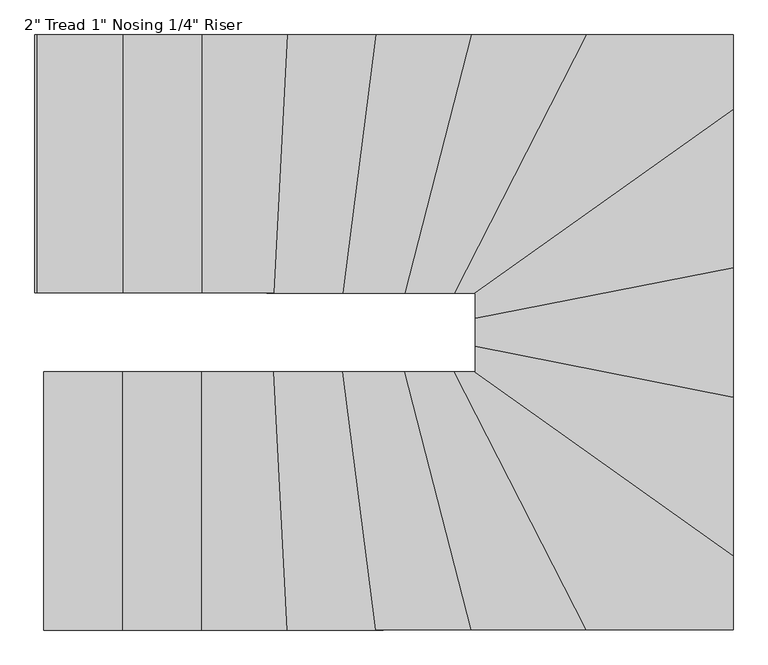
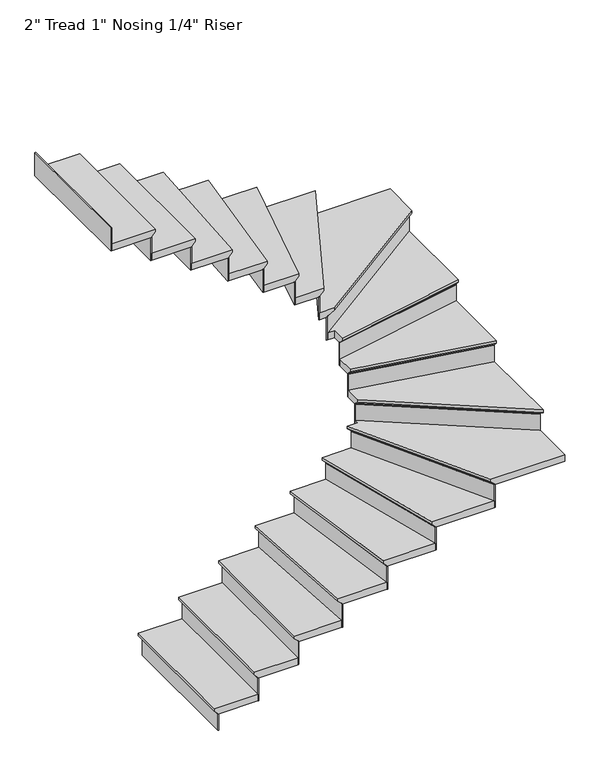
"""IFC4 building model written with IfcOpenShell, lengths in millimetres: stair flight geometry."""

import ifcopenshell
import ifcopenshell.guid

model = None  # the IFC model being written
_history = None  # IfcOwnerHistory: only IFC2X3 demands one
_inside = {}  # id of a spatial element -> (the spatial element, [elements in it])
_under = {}  # id of a project, library or spatial element -> (it, [spatial elements below it])
_declared = {}  # id of a project -> (the project, [libraries it declares])
_typed = {}  # id of a type object -> (the type object, [elements of that type])
_made_of = {}  # id of a material, layer set ... -> (it, [elements and type objects made of it])


def new_model(schema):
    """Start an empty IFC model of exactly this schema.

    Asked for "IFC4X3", IfcOpenShell would pick the latest addendum, in which some entities
    have other attributes; the version numbers below select the first issue.
    IFC2X3 requires an IfcOwnerHistory on every rooted entity: one is made here for all.
    """
    global model, _history
    if schema == "IFC4X3":
        model = ifcopenshell.file(schema_version=(4, 3, 0, 0))
    else:
        model = ifcopenshell.file(schema=schema)
    _inside.clear()
    _under.clear()
    _declared.clear()
    _typed.clear()
    _made_of.clear()
    _history = None
    if model.schema == "IFC2X3":
        org = make("IfcOrganization", Name="unknown")
        user = make(
            "IfcPersonAndOrganization",
            ThePerson=make("IfcPerson", FamilyName="unknown"),
            TheOrganization=org,
        )
        app = make(
            "IfcApplication",
            ApplicationDeveloper=org,
            Version="unknown",
            ApplicationFullName="unknown",
            ApplicationIdentifier="unknown",
        )
        _history = make(
            "IfcOwnerHistory",
            OwningUser=user,
            OwningApplication=app,
            ChangeAction="ADDED",
            CreationDate=0,
        )
    return model


def make(cls, **values):
    """One entity of the class cls with the attributes given. An attribute that is None is left unset."""
    return model.create_entity(
        cls, **{name: value for name, value in values.items() if value is not None}
    )


def rooted(cls, **values):
    """An entity with a GlobalId (a new one), such as an element, a storey or a relation."""
    return make(cls, GlobalId=ifcopenshell.guid.new(), OwnerHistory=_history, **values)


def si_unit(unit_type, name, prefix=None):
    """IfcSIUnit, for example si_unit("LENGTHUNIT", "METRE", prefix="MILLI")."""
    return make("IfcSIUnit", UnitType=unit_type, Prefix=prefix, Name=name)


def assignment(units):
    """IfcUnitAssignment: the units of a project."""
    return None if units is None else make("IfcUnitAssignment", Units=units)


def point(xyz):
    """IfcCartesianPoint."""
    return None if xyz is None else make("IfcCartesianPoint", Coordinates=xyz)


def direction(xyz):
    """IfcDirection."""
    return None if xyz is None else make("IfcDirection", DirectionRatios=xyz)


def frame(location, z_axis=None, x_axis=None):
    """IfcAxis2Placement3D, a coordinate frame: its origin and axes. An axis left out is left unset."""
    return make(
        "IfcAxis2Placement3D",
        Location=point(location),
        Axis=direction(z_axis),
        RefDirection=direction(x_axis),
    )


def origin():
    """The frame at (0, 0, 0) with its axes left unset."""
    return frame((0.0, 0.0, 0.0))


def place(relative_to, where):
    """IfcLocalPlacement: puts the frame where relative to a parent placement (None: the world)."""
    return make(
        "IfcLocalPlacement", PlacementRelTo=relative_to, RelativePlacement=where
    )


def context(
    kind, dimensions, precision=None, world=None, true_north=None, identifier=None
):
    """IfcGeometricRepresentationContext, for example the 3D "Model" context."""
    return make(
        "IfcGeometricRepresentationContext",
        ContextIdentifier=identifier,
        ContextType=kind,
        CoordinateSpaceDimension=dimensions,
        Precision=precision,
        WorldCoordinateSystem=world,
        TrueNorth=true_north,
    )


def project(units=None, contexts=None):
    """IfcProject with its units and contexts."""
    return rooted(
        "IfcProject",
        Name="project",
        RepresentationContexts=contexts,
        UnitsInContext=assignment(units),
    )


def spatial(cls, under=None, at=None, **own):
    """A site, building, storey or space (cls), placed at a placement, below another one or the project."""
    s = rooted(cls, ObjectPlacement=at, **own)
    if under is not None:
        _under.setdefault(under.id(), (under, []))[1].append(s)
    return s


def faces_of(points, faces, orient=None, outer=None):
    """IfcFace entities. A face is a list of loops; a loop is a list of indices into points, from 0.

    orient and outer hold one flag for each loop. By default every Orientation is true, the
    first loop of a face is its IfcFaceOuterBound and the others are IfcFaceBound.
    """
    made = []
    for i, loops in enumerate(faces):
        bounds = []
        for j, loop in enumerate(loops):
            is_outer = j == 0 if outer is None else outer[i][j]
            bounds.append(
                make(
                    "IfcFaceOuterBound" if is_outer else "IfcFaceBound",
                    Bound=make("IfcPolyLoop", Polygon=[points[k] for k in loop]),
                    Orientation=True if orient is None else orient[i][j],
                )
            )
        made.append(make("IfcFace", Bounds=bounds))
    return made


def faceted_brep(points, faces, orient=None, outer=None, voids=None):
    """IfcFacetedBrep: a solid bounded by flat faces; with voids (closed shells), ...WithVoids."""
    shared = [point(p) for p in points]
    hull = make("IfcClosedShell", CfsFaces=faces_of(shared, faces, orient, outer))
    if voids is None:
        return make("IfcFacetedBrep", Outer=hull)
    return make(
        "IfcFacetedBrepWithVoids",
        Outer=hull,
        Voids=[
            make(cls, CfsFaces=faces_of(shared, fs, o, b)) for cls, fs, o, b in voids
        ],
    )


def shape(context_of_items, identifier, shape_type, items):
    """IfcShapeRepresentation: the items that make up one representation, for example the "Body"."""
    return make(
        "IfcShapeRepresentation",
        ContextOfItems=context_of_items,
        RepresentationIdentifier=identifier,
        RepresentationType=shape_type,
        Items=items,
    )


def source(mapping_origin, context_of_items, identifier, shape_type, items):
    """IfcRepresentationMap: a shape defined once, which mapped items show again and again."""
    return make(
        "IfcRepresentationMap",
        MappingOrigin=mapping_origin,
        MappedRepresentation=shape(context_of_items, identifier, shape_type, items),
    )


def transform(
    local_origin,
    x_axis=None,
    y_axis=None,
    z_axis=None,
    scale=None,
    scale2=None,
    scale3=None,
    uniform=True,
):
    """IfcCartesianTransformationOperator3D, or its non-uniform kind. x_axis, y_axis, z_axis: its Axis1, 2, 3."""
    if uniform:
        return make(
            "IfcCartesianTransformationOperator3D",
            Axis1=direction(x_axis),
            Axis2=direction(y_axis),
            LocalOrigin=point(local_origin),
            Scale=scale,
            Axis3=direction(z_axis),
        )
    return make(
        "IfcCartesianTransformationOperator3DnonUniform",
        Axis1=direction(x_axis),
        Axis2=direction(y_axis),
        LocalOrigin=point(local_origin),
        Scale=scale,
        Axis3=direction(z_axis),
        Scale2=scale2,
        Scale3=scale3,
    )


def mapped(mapping_source, mapping_target):
    """IfcMappedItem: shows the shape of a source again, moved by a transform."""
    return make(
        "IfcMappedItem", MappingSource=mapping_source, MappingTarget=mapping_target
    )


def made_of(thing, what):
    """Note that an element or type object is made of a material, layer set ...; save() writes the relation."""
    if what is not None:
        _made_of.setdefault(what.id(), (what, []))[1].append(thing)
    return thing


def element(
    cls,
    number,
    at=None,
    inside=None,
    cuts=None,
    type_object=None,
    material=None,
    context=None,
    identifier="Body",
    shape_type=None,
    held_by="IfcProductDefinitionShape",
    body=None,
    shapes=None,
    **own,
):
    """One element of the class cls, such as IfcWall. Its Tag is "e" and its number.

    at: its placement. inside: the storey or other place that contains it. cuts: it is an
    opening in that element (IfcRelVoidsElement). A single representation is given by context,
    identifier, shape_type and body (its items); several are given by shapes. held_by: the class
    of the entity that holds the representations. save() writes the other relations.
    """
    e = rooted(cls, Tag="e%d" % number, ObjectPlacement=at, **own)
    if body is not None:
        shapes = [shape(context, identifier, shape_type, body)]
    if shapes is not None:
        e.Representation = make(held_by, Representations=shapes)
    if inside is not None:
        _inside.setdefault(inside.id(), (inside, []))[1].append(e)
    if cuts is not None:
        rooted(
            "IfcRelVoidsElement", RelatingBuildingElement=cuts, RelatedOpeningElement=e
        )
    if type_object is not None:
        _typed.setdefault(type_object.id(), (type_object, []))[1].append(e)
    return made_of(e, material)


def aggregate(whole, parts):
    """IfcRelAggregates: a whole, such as a stair, and the parts it consists of."""
    return rooted("IfcRelAggregates", RelatingObject=whole, RelatedObjects=parts)


def save(model, path):
    """Write the relations noted so far, then the file.

    IfcRelAggregates (storeys below a building ...), IfcRelContainedInSpatialStructure (elements
    in a storey), IfcRelDefinesByType, IfcRelAssociatesMaterial and IfcRelDeclares: one each for
    every whole, place, type object, material and project.
    """
    for whole, parts in _under.values():
        aggregate(whole, parts)
    for where, things in _inside.values():
        rooted(
            "IfcRelContainedInSpatialStructure",
            RelatedElements=things,
            RelatingStructure=where,
        )
    for kind, things in _typed.values():
        rooted("IfcRelDefinesByType", RelatedObjects=things, RelatingType=kind)
    for what, things in _made_of.values():
        rooted("IfcRelAssociatesMaterial", RelatedObjects=things, RelatingMaterial=what)
    for by, libraries in _declared.values():
        rooted("IfcRelDeclares", RelatingContext=by, RelatedDefinitions=libraries)
    model.write(path)


def stair_flight_c1eb027c(model_context):
    return source(origin(), model_context, "Body", "Brep", [
        faceted_brep([(-16321.7832832, 2938.4294183, 150.2833333), (-16321.7832832, 2938.4294183, 169.3333333), (-16321.7832832, 3852.8294183, 169.3333333), (-16321.7832832, 3852.8294183, 150.2833333), (-16296.3832832, 2938.4294183, 124.8833333), (-16296.3832832, 3852.8294183, 124.8833333), (-16016.9832832, 2938.4294183, 169.3333333), (-16016.9832832, 3852.8294183, 169.3333333), (-16296.3832832, 3852.8294183, 118.5333333), (-16016.9832832, 3852.8294183, 118.5333333), (-16016.9832832, 2938.4294183, 118.5333333), (-16296.3832832, 2938.4294183, 118.5333333)], [[[0, 1, 2, 3]], [[4, 0, 3, 5]], [[2, 1, 6, 7]], [[8, 9, 10, 11]], [[2, 7, 9, 8, 5, 3]], [[8, 11, 4, 5]], [[6, 1, 0, 4, 11, 10]], [[7, 6, 10, 9]]]),
        faceted_brep([(-16296.3832832, 2938.4294183, 118.5333333), (-16296.3832832, 2938.4294183, 0.0), (-16290.0332832, 2938.4294183, 0.0), (-16290.0332832, 2938.4294183, 118.5333333), (-16296.3832832, 3852.8294183, 118.5333333), (-16290.0332832, 3852.8294183, 118.5333333), (-16290.0332832, 3852.8294183, 0.0), (-16296.3832832, 3852.8294183, 0.0)], [[[0, 1, 2, 3]], [[4, 5, 6, 7]], [[1, 0, 4, 7]], [[2, 1, 7, 6]], [[3, 2, 6, 5]], [[0, 3, 5, 4]]]),
        faceted_brep([(-16016.9832832, 2938.4294183, 287.8666667), (-16016.9832832, 2938.4294183, 118.5333333), (-16010.6332832, 2938.4294183, 118.5333333), (-16010.6332832, 2938.4294183, 287.8666667), (-16016.9832832, 3852.8294183, 287.8666667), (-16010.6332832, 3852.8294183, 287.8666667), (-16010.6332832, 3852.8294183, 118.5333333), (-16016.9832832, 3852.8294183, 118.5333333)], [[[0, 1, 2, 3]], [[4, 5, 6, 7]], [[1, 0, 4, 7]], [[2, 1, 7, 6]], [[3, 2, 6, 5]], [[0, 3, 5, 4]]]),
        faceted_brep([(-16042.3832832, 3852.8294183, 338.6666667), (-16042.3832832, 2938.4294183, 338.6666667), (-15737.5832832, 2938.4294183, 338.6666667), (-15737.5832832, 3852.8294183, 338.6666667), (-16016.9832832, 3852.8294183, 287.8666667), (-15737.5832832, 3852.8294183, 287.8666667), (-15737.5832832, 2938.4294183, 287.8666667), (-16016.9832832, 2938.4294183, 287.8666667), (-16016.9832832, 3852.8294183, 294.2166667), (-16042.3832832, 3852.8294183, 319.6166667), (-16016.9832832, 2938.4294183, 294.2166667), (-16042.3832832, 2938.4294183, 319.6166667)], [[[0, 1, 2, 3]], [[4, 5, 6, 7]], [[0, 3, 5, 4, 8, 9]], [[4, 7, 10, 8]], [[2, 1, 11, 10, 7, 6]], [[3, 2, 6, 5]], [[11, 1, 0, 9]], [[10, 11, 9, 8]]]),
        faceted_brep([(-15737.5832832, 2938.4294183, 457.2), (-15737.5832832, 2938.4294183, 287.8666667), (-15731.2332832, 2938.4294183, 287.8666667), (-15731.2332832, 2938.4294183, 457.2), (-15737.5832832, 3852.8294183, 457.2), (-15731.2332832, 3852.8294183, 457.2), (-15731.2332832, 3852.8294183, 287.8666667), (-15737.5832832, 3852.8294183, 287.8666667)], [[[0, 1, 2, 3]], [[4, 5, 6, 7]], [[1, 0, 4, 7]], [[2, 1, 7, 6]], [[3, 2, 6, 5]], [[0, 3, 5, 4]]]),
        faceted_brep([(-15762.9832832, 3852.8294183, 508.0), (-15762.9832832, 2938.4294183, 508.0), (-15434.3818513, 2938.4294183, 508.0), (-15481.9161218, 3852.8294183, 508.0), (-15737.5832832, 3852.8294183, 457.2), (-15481.9161218, 3852.8294183, 457.2), (-15434.3818513, 2938.4294183, 457.2), (-15737.5832832, 2938.4294183, 457.2), (-15737.5832832, 3852.8294183, 463.55), (-15762.9832832, 3852.8294183, 488.95), (-15737.5832832, 2938.4294183, 463.55), (-15762.9832832, 2938.4294183, 488.95)], [[[0, 1, 2, 3]], [[4, 5, 6, 7]], [[0, 3, 5, 4, 8, 9]], [[4, 7, 10, 8]], [[2, 1, 11, 10, 7, 6]], [[3, 2, 6, 5]], [[11, 1, 0, 9]], [[10, 11, 9, 8]]]),
        faceted_brep([(-15434.3818513, 2938.4294183, 626.5333333), (-15434.3818513, 2938.4294183, 457.2), (-15428.0232772, 2938.4294183, 457.2), (-15428.0232772, 2938.4294183, 626.5333333), (-15481.9161218, 3852.8294183, 626.5333333), (-15475.5575476, 3852.8294183, 626.5333333), (-15475.5575476, 3852.8294183, 457.2), (-15481.9161218, 3852.8294183, 457.2)], [[[0, 1, 2, 3]], [[4, 5, 6, 7]], [[1, 0, 4, 7]], [[2, 1, 7, 6]], [[3, 2, 6, 5]], [[0, 3, 5, 4]]]),
        faceted_brep([(-15507.3504184, 3852.8294183, 677.3333333), (-15459.816148, 2938.4294183, 677.3333333), (-15119.3933703, 2938.4294183, 677.3333333), (-15237.7494219, 3852.8294183, 677.3333333), (-15481.9161218, 3852.8294183, 626.5333333), (-15237.7494219, 3852.8294183, 626.5333333), (-15119.3933703, 2938.4294183, 626.5333333), (-15434.3818513, 2938.4294183, 626.5333333), (-15481.9161218, 3852.8294183, 632.8833333), (-15507.3504184, 3852.8294183, 658.2833333), (-15434.3818513, 2938.4294183, 632.8833333), (-15459.816148, 2938.4294183, 658.2833333)], [[[0, 1, 2, 3]], [[4, 5, 6, 7]], [[0, 3, 5, 4, 8, 9]], [[4, 7, 10, 8]], [[2, 1, 11, 10, 7, 6]], [[3, 2, 6, 5]], [[11, 1, 0, 9]], [[10, 11, 9, 8]]]),
        faceted_brep([(-15119.3933703, 2938.4294183, 795.8666667), (-15119.3933703, 2938.4294183, 626.5333333), (-15112.9903985, 2938.4294183, 626.5333333), (-15112.9903985, 2938.4294183, 795.8666667), (-15237.7494219, 3852.8294183, 795.8666667), (-15231.3464501, 3852.8294183, 795.8666667), (-15231.3464501, 3852.8294183, 626.5333333), (-15237.7494219, 3852.8294183, 626.5333333)], [[[0, 1, 2, 3]], [[4, 5, 6, 7]], [[1, 0, 4, 7]], [[2, 1, 7, 6]], [[3, 2, 6, 5]], [[0, 3, 5, 4]]]),
        faceted_brep([(-15263.361309, 3852.8294183, 846.6666667), (-15145.0052574, 2938.4294183, 846.6666667), (-14780.991752, 2938.4294183, 846.6666667), (-15016.1221995, 3852.8294183, 846.6666667), (-15237.7494219, 3852.8294183, 795.8666667), (-15016.1221995, 3852.8294183, 795.8666667), (-14780.991752, 2938.4294183, 795.8666667), (-15119.3933703, 2938.4294183, 795.8666667), (-15237.7494219, 3852.8294183, 802.2166667), (-15263.361309, 3852.8294183, 827.6166667), (-15119.3933703, 2938.4294183, 802.2166667), (-15145.0052574, 2938.4294183, 827.6166667)], [[[0, 1, 2, 3]], [[4, 5, 6, 7]], [[0, 3, 5, 4, 8, 9]], [[4, 7, 10, 8]], [[2, 1, 11, 10, 7, 6]], [[3, 2, 6, 5]], [[11, 1, 0, 9]], [[10, 11, 9, 8]]]),
        faceted_brep([(-14780.991752, 2938.4294183, 965.2), (-14780.991752, 2938.4294183, 795.8666667), (-14774.4351752, 2938.4294183, 795.8666667), (-14774.4351752, 2938.4294183, 965.2), (-15016.1221995, 3852.8294183, 965.2), (-15009.5656226, 3852.8294183, 965.2), (-15009.5656226, 3852.8294183, 795.8666667), (-15016.1221995, 3852.8294183, 795.8666667)], [[[0, 1, 2, 3]], [[4, 5, 6, 7]], [[1, 0, 4, 7]], [[2, 1, 7, 6]], [[3, 2, 6, 5]], [[0, 3, 5, 4]]]),
        faceted_brep([(-15042.3485069, 3852.8294183, 1016.0), (-14807.2180595, 2938.4294183, 1016.0), (-14370.950942, 2938.4294183, 1016.0), (-14839.7755634, 3852.8294183, 1016.0), (-15016.1221995, 3852.8294183, 965.2), (-14839.7755634, 3852.8294183, 965.2), (-14370.950942, 2938.4294183, 965.2), (-14780.991752, 2938.4294183, 965.2), (-15016.1221995, 3852.8294183, 971.55), (-15042.3485069, 3852.8294183, 996.95), (-14780.991752, 2938.4294183, 971.55), (-14807.2180595, 2938.4294183, 996.95)], [[[0, 1, 2, 3]], [[4, 5, 6, 7]], [[0, 3, 5, 4, 8, 9]], [[4, 7, 10, 8]], [[2, 1, 11, 10, 7, 6]], [[3, 2, 6, 5]], [[11, 1, 0, 9]], [[10, 11, 9, 8]]]),
        faceted_brep([(-14370.950942, 2938.4294183, 1134.5333333), (-14370.950942, 2938.4294183, 965.2), (-14363.8149589, 2938.4294183, 965.2), (-14363.8149589, 2938.4294183, 1134.5333333), (-14839.7755634, 3852.8294183, 1134.5333333), (-14832.6395802, 3852.8294183, 1134.5333333), (-14832.6395802, 3852.8294183, 965.2), (-14839.7755634, 3852.8294183, 965.2)], [[[0, 1, 2, 3]], [[4, 5, 6, 7]], [[1, 0, 4, 7]], [[2, 1, 7, 6]], [[3, 2, 6, 5]], [[0, 3, 5, 4]]]),
        faceted_brep([(-14794.0515914, 3882.3845011, 1185.3333333), (-14794.0515914, 3852.8294183, 1185.3333333), (-14868.3194959, 3852.8294183, 1185.3333333), (-14399.4948746, 2938.4294183, 1185.3333333), (-13879.6515914, 2938.4294183, 1185.3333333), (-13879.6515914, 3232.110552, 1185.3333333), (-14794.0515914, 3852.8294183, 1134.5333333), (-14794.0515914, 3882.3845011, 1134.5333333), (-13879.6515914, 3232.110552, 1134.5333333), (-13879.6515914, 2938.4294183, 1134.5333333), (-14370.950942, 2938.4294183, 1134.5333333), (-14839.7755634, 3852.8294183, 1134.5333333), (-14839.7755634, 3852.8294183, 1140.8833333), (-14868.3194959, 3852.8294183, 1166.2833333), (-14370.950942, 2938.4294183, 1140.8833333), (-14399.4948746, 2938.4294183, 1166.2833333)], [[[0, 1, 2, 3, 4, 5]], [[6, 7, 8, 9, 10, 11]], [[1, 0, 7, 6]], [[2, 1, 6, 11, 12, 13]], [[11, 10, 14, 12]], [[4, 3, 15, 14, 10, 9]], [[5, 4, 9, 8]], [[0, 5, 8, 7]], [[15, 3, 2, 13]], [[14, 15, 13, 12]]]),
        faceted_brep([(-13879.6515914, 3232.110552, 1303.8666667), (-13879.6515914, 3232.110552, 1134.5333333), (-13879.6515914, 3239.9025268, 1134.5333333), (-13879.6515914, 3239.9025268, 1303.8666667), (-14794.0515914, 3882.3845011, 1303.8666667), (-14794.0515914, 3890.1764759, 1303.8666667), (-14794.0515914, 3890.1764759, 1134.5333333), (-14794.0515914, 3882.3845011, 1134.5333333)], [[[0, 1, 2, 3]], [[4, 5, 6, 7]], [[1, 0, 4, 7]], [[2, 1, 7, 6]], [[3, 2, 6, 5]], [[0, 3, 5, 4]]]),
        faceted_brep([(-14794.0515914, 3851.2166019, 1354.6666667), (-13879.6515914, 3200.9426528, 1354.6666667), (-13879.6515914, 3788.5977319, 1354.6666667), (-14794.0515914, 3968.8385882, 1354.6666667), (-14794.0515914, 3882.3845011, 1303.8666667), (-14794.0515914, 3968.8385882, 1303.8666667), (-13879.6515914, 3788.5977319, 1303.8666667), (-13879.6515914, 3232.110552, 1303.8666667), (-14794.0515914, 3882.3845011, 1310.2166667), (-14794.0515914, 3851.2166019, 1335.6166667), (-13879.6515914, 3232.110552, 1310.2166667), (-13879.6515914, 3200.9426528, 1335.6166667)], [[[0, 1, 2, 3]], [[4, 5, 6, 7]], [[0, 3, 5, 4, 8, 9]], [[4, 7, 10, 8]], [[3, 2, 6, 5]], [[11, 1, 0, 9]], [[10, 11, 9, 8]], [[2, 1, 11, 10, 7, 6]]]),
        faceted_brep([(-13879.6515914, 3788.5977319, 1473.2), (-13879.6515914, 3788.5977319, 1303.8666667), (-13879.6515914, 3795.0699173, 1303.8666667), (-13879.6515914, 3795.0699173, 1473.2), (-14794.0515914, 3968.8385882, 1473.2), (-14794.0515914, 3975.3107736, 1473.2), (-14794.0515914, 3975.3107736, 1303.8666667), (-14794.0515914, 3968.8385882, 1303.8666667)], [[[0, 1, 2, 3]], [[4, 5, 6, 7]], [[1, 0, 4, 7]], [[2, 1, 7, 6]], [[3, 2, 6, 5]], [[0, 3, 5, 4]]]),
        faceted_brep([(-14794.0515914, 3942.9498464, 1524.0), (-13879.6515914, 3762.7089901, 1524.0), (-13879.6515914, 4248.2385882, 1524.0), (-14794.0515914, 4067.9977319, 1524.0), (-14794.0515914, 3968.8385882, 1473.2), (-14794.0515914, 4067.9977319, 1473.2), (-13879.6515914, 4248.2385882, 1473.2), (-13879.6515914, 3788.5977319, 1473.2), (-14794.0515914, 3968.8385882, 1479.55), (-14794.0515914, 3942.9498464, 1504.95), (-13879.6515914, 3788.5977319, 1479.55), (-13879.6515914, 3762.7089901, 1504.95)], [[[0, 1, 2, 3]], [[4, 5, 6, 7]], [[0, 3, 5, 4, 8, 9]], [[4, 7, 10, 8]], [[2, 1, 11, 10, 7, 6]], [[3, 2, 6, 5]], [[11, 1, 0, 9]], [[10, 11, 9, 8]]]),
        faceted_brep([(-13879.6515914, 4248.2385882, 1642.5333333), (-13879.6515914, 4248.2385882, 1473.2), (-13879.6515914, 4254.7107736, 1473.2), (-13879.6515914, 4254.7107736, 1642.5333333), (-14794.0515914, 4067.9977319, 1642.5333333), (-14794.0515914, 4074.4699173, 1642.5333333), (-14794.0515914, 4074.4699173, 1473.2), (-14794.0515914, 4067.9977319, 1473.2)], [[[0, 1, 2, 3]], [[4, 5, 6, 7]], [[1, 0, 4, 7]], [[2, 1, 7, 6]], [[3, 2, 6, 5]], [[0, 3, 5, 4]]]),
        faceted_brep([(-14840.1470659, 4132.2294183, 1693.3333333), (-14794.0515914, 4132.2294183, 1693.3333333), (-14794.0515914, 4042.1089901, 1693.3333333), (-13879.6515914, 4222.3498464, 1693.3333333), (-13879.6515914, 4815.2840829, 1693.3333333), (-14794.0515914, 4132.2294183, 1642.5333333), (-14840.1470659, 4132.2294183, 1642.5333333), (-13879.6515914, 4815.2840829, 1642.5333333), (-13879.6515914, 4248.2385882, 1642.5333333), (-14794.0515914, 4067.9977319, 1642.5333333), (-13879.6515914, 4248.2385882, 1648.8833333), (-14794.0515914, 4067.9977319, 1648.8833333), (-13879.6515914, 4222.3498464, 1674.2833333), (-14794.0515914, 4042.1089901, 1674.2833333)], [[[0, 1, 2, 3, 4]], [[5, 6, 7, 8, 9]], [[1, 0, 6, 5]], [[9, 8, 10, 11]], [[4, 3, 12, 10, 8, 7]], [[0, 4, 7, 6]], [[12, 3, 2, 13]], [[10, 12, 13, 11]], [[2, 1, 5, 9, 11, 13]]]),
        faceted_brep([(-13879.6515914, 4815.2840829, 1811.8666667), (-13879.6515914, 4815.2840829, 1642.5333333), (-13879.6515914, 4823.0760577, 1642.5333333), (-13879.6515914, 4823.0760577, 1811.8666667), (-14840.1470659, 4132.2294183, 1811.8666667), (-14851.1039584, 4132.2294183, 1811.8666667), (-14851.1039584, 4132.2294183, 1642.5333333), (-14840.1470659, 4132.2294183, 1642.5333333)], [[[0, 1, 2, 3]], [[4, 5, 6, 7]], [[1, 0, 4, 7]], [[2, 1, 7, 6]], [[3, 2, 6, 5]], [[0, 3, 5, 4]]]),
        faceted_brep([(-14796.3194959, 4132.2294183, 1862.6666667), (-13879.6515914, 4784.1161838, 1862.6666667), (-13879.6515914, 5046.6294183, 1862.6666667), (-14428.0388071, 5046.6294183, 1862.6666667), (-14896.8634284, 4132.2294183, 1862.6666667), (-14840.1470659, 4132.2294183, 1811.8666667), (-14896.8634284, 4132.2294183, 1811.8666667), (-14428.0388071, 5046.6294183, 1811.8666667), (-13879.6515914, 5046.6294183, 1811.8666667), (-13879.6515914, 4815.2840829, 1811.8666667), (-14840.1470659, 4132.2294183, 1818.2166667), (-14796.3194959, 4132.2294183, 1843.6166667), (-13879.6515914, 4815.2840829, 1818.2166667), (-13879.6515914, 4784.1161838, 1843.6166667)], [[[0, 1, 2, 3, 4]], [[5, 6, 7, 8, 9]], [[0, 4, 6, 5, 10, 11]], [[5, 9, 12, 10]], [[2, 1, 13, 12, 9, 8]], [[4, 3, 7, 6]], [[13, 1, 0, 11]], [[12, 13, 11, 10]], [[3, 2, 8, 7]]]),
        faceted_brep([(-14428.0388071, 5046.6294183, 1981.2), (-14428.0388071, 5046.6294183, 1811.8666667), (-14435.1747902, 5046.6294183, 1811.8666667), (-14435.1747902, 5046.6294183, 1981.2), (-14896.8634284, 4132.2294183, 1981.2), (-14903.9994116, 4132.2294183, 1981.2), (-14903.9994116, 4132.2294183, 1811.8666667), (-14896.8634284, 4132.2294183, 1811.8666667)], [[[0, 1, 2, 3]], [[4, 5, 6, 7]], [[1, 0, 4, 7]], [[2, 1, 7, 6]], [[3, 2, 6, 5]], [[0, 3, 5, 4]]]),
        faceted_brep([(-14868.3194959, 4132.2294183, 2032.0), (-14399.4948746, 5046.6294183, 2032.0), (-14833.444367, 5046.6294183, 2032.0), (-15068.5748144, 4132.2294183, 2032.0), (-14896.8634284, 4132.2294183, 1981.2), (-15068.5748144, 4132.2294183, 1981.2), (-14833.444367, 5046.6294183, 1981.2), (-14428.0388071, 5046.6294183, 1981.2), (-14896.8634284, 4132.2294183, 1987.55), (-14868.3194959, 4132.2294183, 2012.95), (-14428.0388071, 5046.6294183, 1987.55), (-14399.4948746, 5046.6294183, 2012.95)], [[[0, 1, 2, 3]], [[4, 5, 6, 7]], [[0, 3, 5, 4, 8, 9]], [[4, 7, 10, 8]], [[2, 1, 11, 10, 7, 6]], [[3, 2, 6, 5]], [[11, 1, 0, 9]], [[10, 11, 9, 8]]]),
        faceted_brep([(-14833.444367, 5046.6294183, 2150.5333333), (-14833.444367, 5046.6294183, 1981.2), (-14840.0009438, 5046.6294183, 1981.2), (-14840.0009438, 5046.6294183, 2150.5333333), (-15068.5748144, 4132.2294183, 2150.5333333), (-15075.1313912, 4132.2294183, 2150.5333333), (-15075.1313912, 4132.2294183, 1981.2), (-15068.5748144, 4132.2294183, 1981.2)], [[[0, 1, 2, 3]], [[4, 5, 6, 7]], [[1, 0, 4, 7]], [[2, 1, 7, 6]], [[3, 2, 6, 5]], [[0, 3, 5, 4]]]),
        faceted_brep([(-15042.3485069, 4132.2294183, 2201.3333333), (-14807.2180595, 5046.6294183, 2201.3333333), (-15170.6171445, 5046.6294183, 2201.3333333), (-15288.9731962, 4132.2294183, 2201.3333333), (-15068.5748144, 4132.2294183, 2150.5333333), (-15288.9731962, 4132.2294183, 2150.5333333), (-15170.6171445, 5046.6294183, 2150.5333333), (-14833.444367, 5046.6294183, 2150.5333333), (-15068.5748144, 4132.2294183, 2156.8833333), (-15042.3485069, 4132.2294183, 2182.2833333), (-14833.444367, 5046.6294183, 2156.8833333), (-14807.2180595, 5046.6294183, 2182.2833333)], [[[0, 1, 2, 3]], [[4, 5, 6, 7]], [[0, 3, 5, 4, 8, 9]], [[4, 7, 10, 8]], [[2, 1, 11, 10, 7, 6]], [[3, 2, 6, 5]], [[11, 1, 0, 9]], [[10, 11, 9, 8]]]),
        faceted_brep([(-15170.6171445, 5046.6294183, 2319.8666667), (-15170.6171445, 5046.6294183, 2150.5333333), (-15177.0201163, 5046.6294183, 2150.5333333), (-15177.0201163, 5046.6294183, 2319.8666667), (-15288.9731962, 4132.2294183, 2319.8666667), (-15295.3761679, 4132.2294183, 2319.8666667), (-15295.3761679, 4132.2294183, 2150.5333333), (-15288.9731962, 4132.2294183, 2150.5333333)], [[[0, 1, 2, 3]], [[4, 5, 6, 7]], [[1, 0, 4, 7]], [[2, 1, 7, 6]], [[3, 2, 6, 5]], [[0, 3, 5, 4]]]),
        faceted_brep([(-15263.361309, 4132.2294183, 2370.6666667), (-15145.0052574, 5046.6294183, 2370.6666667), (-15485.2504447, 5046.6294183, 2370.6666667), (-15532.7847151, 4132.2294183, 2370.6666667), (-15288.9731962, 4132.2294183, 2319.8666667), (-15532.7847151, 4132.2294183, 2319.8666667), (-15485.2504447, 5046.6294183, 2319.8666667), (-15170.6171445, 5046.6294183, 2319.8666667), (-15288.9731962, 4132.2294183, 2326.2166667), (-15263.361309, 4132.2294183, 2351.6166667), (-15170.6171445, 5046.6294183, 2326.2166667), (-15145.0052574, 5046.6294183, 2351.6166667)], [[[0, 1, 2, 3]], [[4, 5, 6, 7]], [[0, 3, 5, 4, 8, 9]], [[4, 7, 10, 8]], [[2, 1, 11, 10, 7, 6]], [[3, 2, 6, 5]], [[11, 1, 0, 9]], [[10, 11, 9, 8]]]),
        faceted_brep([(-15485.2504447, 5046.6294183, 2489.2), (-15485.2504447, 5046.6294183, 2319.8666667), (-15491.6090188, 5046.6294183, 2319.8666667), (-15491.6090188, 5046.6294183, 2489.2), (-15532.7847151, 4132.2294183, 2489.2), (-15539.1432892, 4132.2294183, 2489.2), (-15539.1432892, 4132.2294183, 2319.8666667), (-15532.7847151, 4132.2294183, 2319.8666667)], [[[0, 1, 2, 3]], [[4, 5, 6, 7]], [[1, 0, 4, 7]], [[2, 1, 7, 6]], [[3, 2, 6, 5]], [[0, 3, 5, 4]]]),
        faceted_brep([(-15507.3504184, 4132.2294183, 2540.0), (-15459.816148, 5046.6294183, 2540.0), (-15788.3832832, 5046.6294183, 2540.0), (-15788.3832832, 4132.2294183, 2540.0), (-15532.7847151, 4132.2294183, 2489.2), (-15788.3832832, 4132.2294183, 2489.2), (-15788.3832832, 5046.6294183, 2489.2), (-15485.2504447, 5046.6294183, 2489.2), (-15532.7847151, 4132.2294183, 2495.55), (-15507.3504184, 4132.2294183, 2520.95), (-15485.2504447, 5046.6294183, 2495.55), (-15459.816148, 5046.6294183, 2520.95)], [[[0, 1, 2, 3]], [[4, 5, 6, 7]], [[0, 3, 5, 4, 8, 9]], [[4, 7, 10, 8]], [[2, 1, 11, 10, 7, 6]], [[3, 2, 6, 5]], [[11, 1, 0, 9]], [[10, 11, 9, 8]]]),
        faceted_brep([(-15788.3832832, 5046.6294183, 2658.5333333), (-15788.3832832, 5046.6294183, 2489.2), (-15794.7332832, 5046.6294183, 2489.2), (-15794.7332832, 5046.6294183, 2658.5333333), (-15788.3832832, 4132.2294183, 2658.5333333), (-15794.7332832, 4132.2294183, 2658.5333333), (-15794.7332832, 4132.2294183, 2489.2), (-15788.3832832, 4132.2294183, 2489.2)], [[[0, 1, 2, 3]], [[4, 5, 6, 7]], [[1, 0, 4, 7]], [[2, 1, 7, 6]], [[3, 2, 6, 5]], [[0, 3, 5, 4]]]),
        faceted_brep([(-15762.9832832, 4132.2294183, 2709.3333333), (-15762.9832832, 5046.6294183, 2709.3333333), (-16067.7832832, 5046.6294183, 2709.3333333), (-16067.7832832, 4132.2294183, 2709.3333333), (-15788.3832832, 4132.2294183, 2658.5333333), (-16067.7832832, 4132.2294183, 2658.5333333), (-16067.7832832, 5046.6294183, 2658.5333333), (-15788.3832832, 5046.6294183, 2658.5333333), (-15788.3832832, 4132.2294183, 2664.8833333), (-15762.9832832, 4132.2294183, 2690.2833333), (-15788.3832832, 5046.6294183, 2664.8833333), (-15762.9832832, 5046.6294183, 2690.2833333)], [[[0, 1, 2, 3]], [[4, 5, 6, 7]], [[0, 3, 5, 4, 8, 9]], [[4, 7, 10, 8]], [[2, 1, 11, 10, 7, 6]], [[3, 2, 6, 5]], [[11, 1, 0, 9]], [[10, 11, 9, 8]]]),
        faceted_brep([(-16067.7832832, 5046.6294183, 2827.8666667), (-16067.7832832, 5046.6294183, 2658.5333333), (-16074.1332832, 5046.6294183, 2658.5333333), (-16074.1332832, 5046.6294183, 2827.8666667), (-16067.7832832, 4132.2294183, 2827.8666667), (-16074.1332832, 4132.2294183, 2827.8666667), (-16074.1332832, 4132.2294183, 2658.5333333), (-16067.7832832, 4132.2294183, 2658.5333333)], [[[0, 1, 2, 3]], [[4, 5, 6, 7]], [[1, 0, 4, 7]], [[2, 1, 7, 6]], [[3, 2, 6, 5]], [[0, 3, 5, 4]]]),
        faceted_brep([(-16347.1832832, 5046.6294183, 2997.2), (-16347.1832832, 5046.6294183, 2827.8666667), (-16353.5332832, 5046.6294183, 2827.8666667), (-16353.5332832, 5046.6294183, 2997.2), (-16347.1832832, 4132.2294183, 2997.2), (-16353.5332832, 4132.2294183, 2997.2), (-16353.5332832, 4132.2294183, 2827.8666667), (-16347.1832832, 4132.2294183, 2827.8666667)], [[[0, 1, 2, 3]], [[4, 5, 6, 7]], [[1, 0, 4, 7]], [[2, 1, 7, 6]], [[3, 2, 6, 5]], [[0, 3, 5, 4]]]),
        faceted_brep([(-16042.3832832, 4132.2294183, 2878.6666667), (-16042.3832832, 5046.6294183, 2878.6666667), (-16347.1832832, 5046.6294183, 2878.6666667), (-16347.1832832, 4132.2294183, 2878.6666667), (-16067.7832832, 4132.2294183, 2827.8666667), (-16347.1832832, 4132.2294183, 2827.8666667), (-16347.1832832, 5046.6294183, 2827.8666667), (-16067.7832832, 5046.6294183, 2827.8666667), (-16067.7832832, 4132.2294183, 2834.2166667), (-16042.3832832, 4132.2294183, 2859.6166667), (-16067.7832832, 5046.6294183, 2834.2166667), (-16042.3832832, 5046.6294183, 2859.6166667)], [[[0, 1, 2, 3]], [[4, 5, 6, 7]], [[0, 3, 5, 4, 8, 9]], [[4, 7, 10, 8]], [[2, 1, 11, 10, 7, 6]], [[3, 2, 6, 5]], [[11, 1, 0, 9]], [[10, 11, 9, 8]]]),
    ])


if __name__ == "__main__":
    model = new_model("IFC4")
    model_context = context("Model", 3, world=origin())
    ifc_project = project(units=[si_unit("LENGTHUNIT", "METRE", prefix="MILLI")], contexts=[model_context])
    site = spatial("IfcSite", under=ifc_project)
    building = spatial("IfcBuilding", under=site)
    placement = place(None, origin())
    stair_flight_shape = stair_flight_c1eb027c(model_context)
    element("IfcStairFlight", 1, ObjectType="2\" Tread 1\" Nosing 1/4\" Riser", at=placement, inside=building, context=model_context, shape_type="MappedRepresentation", body=[
        mapped(stair_flight_shape, transform((0.0, 0.0, 0.0), x_axis=(1.0, 0.0, 0.0), y_axis=(0.0, 1.0, 0.0), z_axis=(0.0, 0.0, 1.0))),
    ])
    save(model, "model.ifc")
